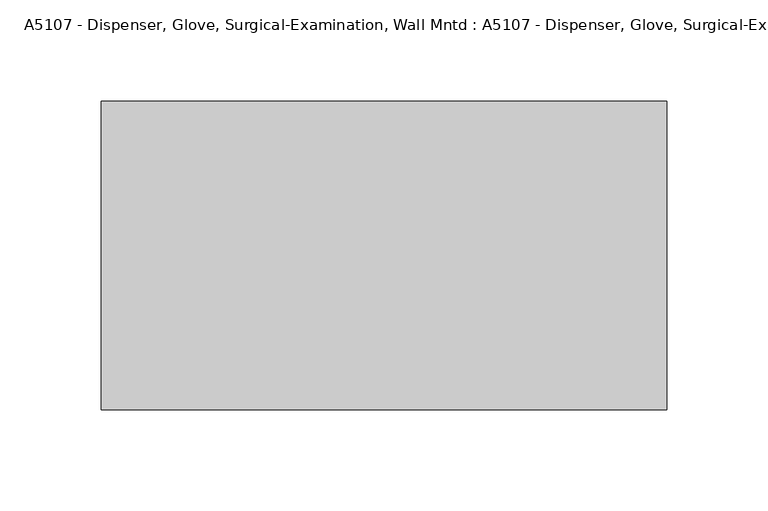
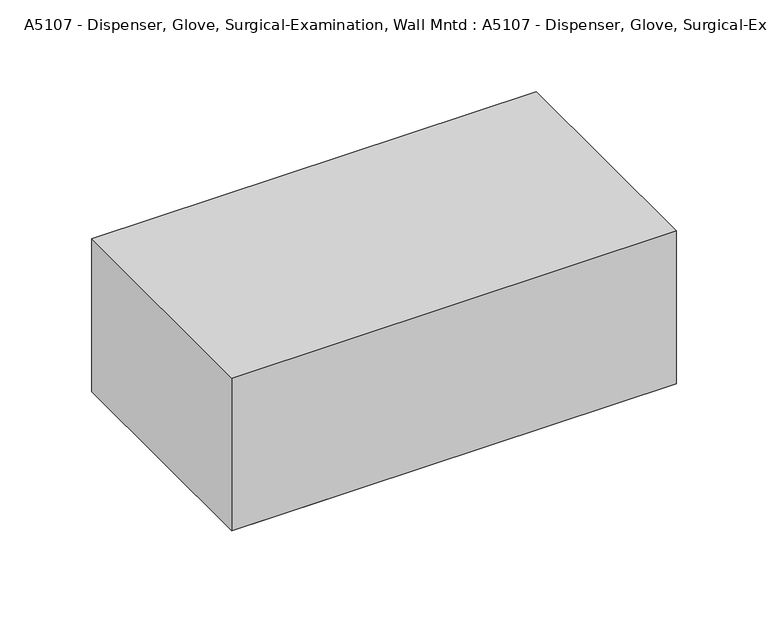
"""IFC4 building model written with IfcOpenShell, lengths in millimetres: proxy geometry, A5107 - Dispenser, Glove, Surgical-Examination, Wall Mntd : A5107 - Dispenser, Glove, Surgical-Examination, Wall Mntd."""

import ifcopenshell
import ifcopenshell.guid

model = None  # the IFC model being written
_history = None  # IfcOwnerHistory: only IFC2X3 demands one
_inside = {}  # id of a spatial element -> (the spatial element, [elements in it])
_under = {}  # id of a project, library or spatial element -> (it, [spatial elements below it])
_declared = {}  # id of a project -> (the project, [libraries it declares])
_typed = {}  # id of a type object -> (the type object, [elements of that type])
_made_of = {}  # id of a material, layer set ... -> (it, [elements and type objects made of it])


def new_model(schema):
    """Start an empty IFC model of exactly this schema.

    Asked for "IFC4X3", IfcOpenShell would pick the latest addendum, in which some entities
    have other attributes; the version numbers below select the first issue.
    IFC2X3 requires an IfcOwnerHistory on every rooted entity: one is made here for all.
    """
    global model, _history
    if schema == "IFC4X3":
        model = ifcopenshell.file(schema_version=(4, 3, 0, 0))
    else:
        model = ifcopenshell.file(schema=schema)
    _inside.clear()
    _under.clear()
    _declared.clear()
    _typed.clear()
    _made_of.clear()
    _history = None
    if model.schema == "IFC2X3":
        org = make("IfcOrganization", Name="unknown")
        user = make(
            "IfcPersonAndOrganization",
            ThePerson=make("IfcPerson", FamilyName="unknown"),
            TheOrganization=org,
        )
        app = make(
            "IfcApplication",
            ApplicationDeveloper=org,
            Version="unknown",
            ApplicationFullName="unknown",
            ApplicationIdentifier="unknown",
        )
        _history = make(
            "IfcOwnerHistory",
            OwningUser=user,
            OwningApplication=app,
            ChangeAction="ADDED",
            CreationDate=0,
        )
    return model


def make(cls, **values):
    """One entity of the class cls with the attributes given. An attribute that is None is left unset."""
    return model.create_entity(
        cls, **{name: value for name, value in values.items() if value is not None}
    )


def rooted(cls, **values):
    """An entity with a GlobalId (a new one), such as an element, a storey or a relation."""
    return make(cls, GlobalId=ifcopenshell.guid.new(), OwnerHistory=_history, **values)


def si_unit(unit_type, name, prefix=None):
    """IfcSIUnit, for example si_unit("LENGTHUNIT", "METRE", prefix="MILLI")."""
    return make("IfcSIUnit", UnitType=unit_type, Prefix=prefix, Name=name)


def assignment(units):
    """IfcUnitAssignment: the units of a project."""
    return None if units is None else make("IfcUnitAssignment", Units=units)


def point(xyz):
    """IfcCartesianPoint."""
    return None if xyz is None else make("IfcCartesianPoint", Coordinates=xyz)


def direction(xyz):
    """IfcDirection."""
    return None if xyz is None else make("IfcDirection", DirectionRatios=xyz)


def frame(location, z_axis=None, x_axis=None):
    """IfcAxis2Placement3D, a coordinate frame: its origin and axes. An axis left out is left unset."""
    return make(
        "IfcAxis2Placement3D",
        Location=point(location),
        Axis=direction(z_axis),
        RefDirection=direction(x_axis),
    )


def origin():
    """The frame at (0, 0, 0) with its axes left unset."""
    return frame((0.0, 0.0, 0.0))


def origin_with_axes():
    """The frame at (0, 0, 0) with the z axis (0, 0, 1) and the x axis (1, 0, 0) written out."""
    return frame((0.0, 0.0, 0.0), z_axis=(0.0, 0.0, 1.0), x_axis=(1.0, 0.0, 0.0))


def place(relative_to, where):
    """IfcLocalPlacement: puts the frame where relative to a parent placement (None: the world)."""
    return make(
        "IfcLocalPlacement", PlacementRelTo=relative_to, RelativePlacement=where
    )


def context(
    kind, dimensions, precision=None, world=None, true_north=None, identifier=None
):
    """IfcGeometricRepresentationContext, for example the 3D "Model" context."""
    return make(
        "IfcGeometricRepresentationContext",
        ContextIdentifier=identifier,
        ContextType=kind,
        CoordinateSpaceDimension=dimensions,
        Precision=precision,
        WorldCoordinateSystem=world,
        TrueNorth=true_north,
    )


def project(units=None, contexts=None):
    """IfcProject with its units and contexts."""
    return rooted(
        "IfcProject",
        Name="project",
        RepresentationContexts=contexts,
        UnitsInContext=assignment(units),
    )


def spatial(cls, under=None, at=None, **own):
    """A site, building, storey or space (cls), placed at a placement, below another one or the project."""
    s = rooted(cls, ObjectPlacement=at, **own)
    if under is not None:
        _under.setdefault(under.id(), (under, []))[1].append(s)
    return s


def polyline(points):
    """IfcPolyline through the points."""
    return make("IfcPolyline", Points=[point(p) for p in points])


def outline(outer, holes=None, kind="AREA"):
    """IfcArbitraryClosedProfileDef: a profile drawn as a closed curve; with holes, ...WithVoids."""
    if holes is None:
        return make("IfcArbitraryClosedProfileDef", ProfileType=kind, OuterCurve=outer)
    return make(
        "IfcArbitraryProfileDefWithVoids",
        ProfileType=kind,
        OuterCurve=outer,
        InnerCurves=holes,
    )


def extrude(swept, where, along, depth):
    """IfcExtrudedAreaSolid: the profile swept, set in the frame where, extruded along a direction by depth."""
    return make(
        "IfcExtrudedAreaSolid",
        SweptArea=swept,
        Position=where,
        ExtrudedDirection=direction(along),
        Depth=depth,
    )


def shape(context_of_items, identifier, shape_type, items):
    """IfcShapeRepresentation: the items that make up one representation, for example the "Body"."""
    return make(
        "IfcShapeRepresentation",
        ContextOfItems=context_of_items,
        RepresentationIdentifier=identifier,
        RepresentationType=shape_type,
        Items=items,
    )


def source(mapping_origin, context_of_items, identifier, shape_type, items):
    """IfcRepresentationMap: a shape defined once, which mapped items show again and again."""
    return make(
        "IfcRepresentationMap",
        MappingOrigin=mapping_origin,
        MappedRepresentation=shape(context_of_items, identifier, shape_type, items),
    )


def transform(
    local_origin,
    x_axis=None,
    y_axis=None,
    z_axis=None,
    scale=None,
    scale2=None,
    scale3=None,
    uniform=True,
):
    """IfcCartesianTransformationOperator3D, or its non-uniform kind. x_axis, y_axis, z_axis: its Axis1, 2, 3."""
    if uniform:
        return make(
            "IfcCartesianTransformationOperator3D",
            Axis1=direction(x_axis),
            Axis2=direction(y_axis),
            LocalOrigin=point(local_origin),
            Scale=scale,
            Axis3=direction(z_axis),
        )
    return make(
        "IfcCartesianTransformationOperator3DnonUniform",
        Axis1=direction(x_axis),
        Axis2=direction(y_axis),
        LocalOrigin=point(local_origin),
        Scale=scale,
        Axis3=direction(z_axis),
        Scale2=scale2,
        Scale3=scale3,
    )


def mapped(mapping_source, mapping_target):
    """IfcMappedItem: shows the shape of a source again, moved by a transform."""
    return make(
        "IfcMappedItem", MappingSource=mapping_source, MappingTarget=mapping_target
    )


def made_of(thing, what):
    """Note that an element or type object is made of a material, layer set ...; save() writes the relation."""
    if what is not None:
        _made_of.setdefault(what.id(), (what, []))[1].append(thing)
    return thing


def element(
    cls,
    number,
    at=None,
    inside=None,
    cuts=None,
    type_object=None,
    material=None,
    context=None,
    identifier="Body",
    shape_type=None,
    held_by="IfcProductDefinitionShape",
    body=None,
    shapes=None,
    **own,
):
    """One element of the class cls, such as IfcWall. Its Tag is "e" and its number.

    at: its placement. inside: the storey or other place that contains it. cuts: it is an
    opening in that element (IfcRelVoidsElement). A single representation is given by context,
    identifier, shape_type and body (its items); several are given by shapes. held_by: the class
    of the entity that holds the representations. save() writes the other relations.
    """
    e = rooted(cls, Tag="e%d" % number, ObjectPlacement=at, **own)
    if body is not None:
        shapes = [shape(context, identifier, shape_type, body)]
    if shapes is not None:
        e.Representation = make(held_by, Representations=shapes)
    if inside is not None:
        _inside.setdefault(inside.id(), (inside, []))[1].append(e)
    if cuts is not None:
        rooted(
            "IfcRelVoidsElement", RelatingBuildingElement=cuts, RelatedOpeningElement=e
        )
    if type_object is not None:
        _typed.setdefault(type_object.id(), (type_object, []))[1].append(e)
    return made_of(e, material)


def aggregate(whole, parts):
    """IfcRelAggregates: a whole, such as a stair, and the parts it consists of."""
    return rooted("IfcRelAggregates", RelatingObject=whole, RelatedObjects=parts)


def save(model, path):
    """Write the relations noted so far, then the file.

    IfcRelAggregates (storeys below a building ...), IfcRelContainedInSpatialStructure (elements
    in a storey), IfcRelDefinesByType, IfcRelAssociatesMaterial and IfcRelDeclares: one each for
    every whole, place, type object, material and project.
    """
    for whole, parts in _under.values():
        aggregate(whole, parts)
    for where, things in _inside.values():
        rooted(
            "IfcRelContainedInSpatialStructure",
            RelatedElements=things,
            RelatingStructure=where,
        )
    for kind, things in _typed.values():
        rooted("IfcRelDefinesByType", RelatedObjects=things, RelatingType=kind)
    for what, things in _made_of.values():
        rooted("IfcRelAssociatesMaterial", RelatedObjects=things, RelatingMaterial=what)
    for by, libraries in _declared.values():
        rooted("IfcRelDeclares", RelatingContext=by, RelatedDefinitions=libraries)
    model.write(path)


def a5107_dispenser_glove_surgical_examination_wall_mntd_a5107_9fe0d71b(model_context):
    return source(origin(), model_context, "Body", "SweptSolid", [
        extrude(outline(polyline([(139.7, 76.2), (139.7, -76.2), (-139.7, -76.2), (-139.7, 76.2), (139.7, 76.2)])), origin_with_axes(), (0.0, 0.0, 1.0), 101.6),
        extrude(outline(polyline([(127.0, 76.2), (127.0, -76.2), (-127.0, -76.2), (-127.0, 76.2), (127.0, 76.2)])), origin_with_axes(), (0.0, 0.0, 1.0), 101.6),
    ])


if __name__ == "__main__":
    model = new_model("IFC4")
    model_context = context("Model", 3, world=origin())
    ifc_project = project(units=[si_unit("LENGTHUNIT", "METRE", prefix="MILLI")], contexts=[model_context])
    site = spatial("IfcSite", under=ifc_project)
    building = spatial("IfcBuilding", under=site)
    placement = place(None, origin())
    a5107_dispenser_glove_surgical_examination_wall_mntd_a5107_shape = a5107_dispenser_glove_surgical_examination_wall_mntd_a5107_9fe0d71b(model_context)
    element("IfcBuildingElementProxy", 1, Name="A5107 - Dispenser, Glove, Surgical-Examination, Wall Mntd : A5107 - Dispenser, Glove, Surgical-Examination, Wall Mntd", ObjectType="A5107 - Dispenser, Glove, Surgical-Examination, Wall Mntd : A5107 - Dispenser, Glove, Surgical-Examination, Wall Mntd", at=placement, inside=building, context=model_context, shape_type="MappedRepresentation", body=[
        mapped(a5107_dispenser_glove_surgical_examination_wall_mntd_a5107_shape, transform((0.0, 0.0, 0.0), x_axis=(1.0, 0.0, 0.0), y_axis=(0.0, 1.0, 0.0), z_axis=(0.0, 0.0, 1.0))),
    ])
    save(model, "model.ifc")

# Revit data of these elements
# Type "A5107 - Dispenser, Glove, Surgical-Examination, Wall Mntd : A5107 - Dispenser, Glove, Surgical-Examination, Wall Mntd"
#   Watts2 = "0"
#   Watts1 = "0"
#   Unit_Issue = "EA"
#   UTIL_6_Misc = "-"
#   UTIL_5_NonMedGas = "-"
#   UTIL_4_MiscGas = "-"
#   UTIL_3_MedGas = "-"
#   UTIL_2_Elec = "-"
#   UTIL_1_WaterDrain = "-"
#   Nomenclature = "Dispenser, Glove, Surgical/Examination, Wall Mntd"
#   NSN = "4510"
#   Location [instance default] = ""
#   JSN = "A5107"
#   Fund_Source_VA = "-"
#   Fund_Source_Navy = "C"
#   Fund_Source_Army = "-"
#   Fund_Source_AF = "-"
#   ELEC_Volts2 = "0"
#   ELEC_Volts1 = "0"
#   ELEC_Phase2 = "0"
#   ELEC_Phase1 = "0"
#   ELEC_HertzSwitch = "0"
#   ELEC_HertzDependent = "0"
#   ELEC_Hertz = "0"
#   ELEC_Amps2 = "0"
#   ELEC_Amps1 = "0"
#   DetailDescription = "Examination glove dispenser box for wall mounting. Fabricated of either cold rolled steel with a white baked enamel finish, plastic or acrylic. Provided with wall bracket to facilitate mounting and demounting."
#   CAT_VA = "C"
#   CAT_Navy = "C"
#   CAT_IHS = "-"
#   CAT_Army = "C"
#   CAT_AF = "C"
#   BTUperhour = "0"
#   Weight_IP = 2
#   Default Elevation = 4' - 0"
#   DIM_Width_IP = 0' - 11"
#   DIM_Height_IP = 0' - 6"
#   DIM_Depth_IP = 0' - 4"
#   finish [instance default] = none
#   Assembly Code = ""
# Element 1 (IfcBuildingElementProxy, "A5107 - Dispenser, Glove, Surgical-Examination, Wall Mntd : A5107 - Dispenser, Glove, Surgical-Examination, Wall Mntd")
#   Materials on its faces: "EquipSpace"
# Materials
#   "EquipSpace": class "Unassigned", colour RGB 221 217 195, transparency 0.5
